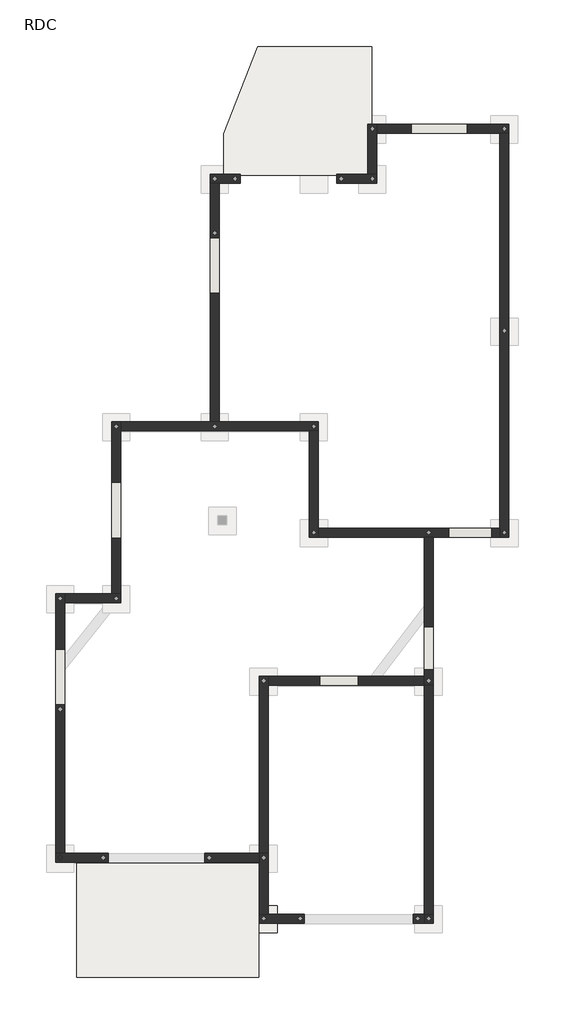
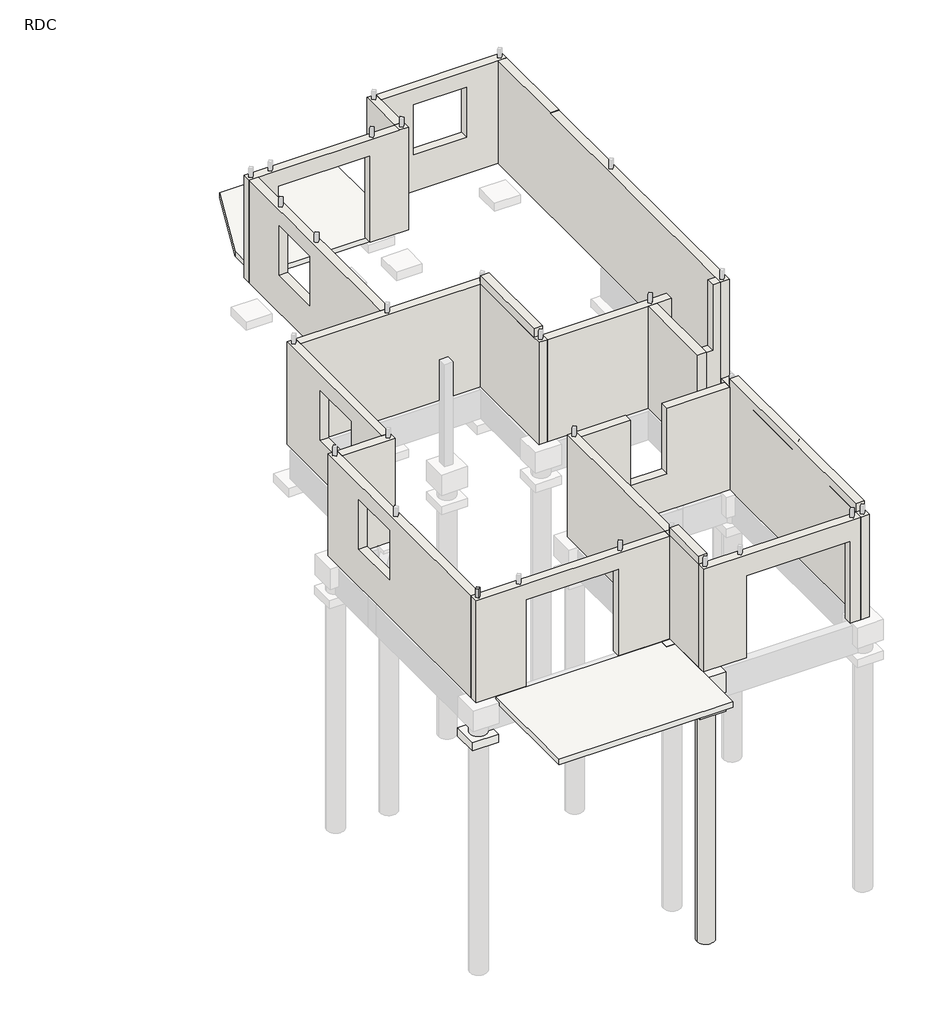
# One storey, part 1 of 5: 20 walls, 5 slabs, 1 column.
"""IFC4 building model written with IfcOpenShell, lengths in millimetres."""

import ifcopenshell
import ifcopenshell.guid

model = None  # the IFC model being written
_history = None  # IfcOwnerHistory: only IFC2X3 demands one
_inside = {}  # id of a spatial element -> (the spatial element, [elements in it])
_under = {}  # id of a project, library or spatial element -> (it, [spatial elements below it])
_declared = {}  # id of a project -> (the project, [libraries it declares])
_typed = {}  # id of a type object -> (the type object, [elements of that type])
_made_of = {}  # id of a material, layer set ... -> (it, [elements and type objects made of it])


def new_model(schema):
    """Start an empty IFC model of exactly this schema.

    Asked for "IFC4X3", IfcOpenShell would pick the latest addendum, in which some entities
    have other attributes; the version numbers below select the first issue.
    IFC2X3 requires an IfcOwnerHistory on every rooted entity: one is made here for all.
    """
    global model, _history
    if schema == "IFC4X3":
        model = ifcopenshell.file(schema_version=(4, 3, 0, 0))
    else:
        model = ifcopenshell.file(schema=schema)
    _inside.clear()
    _under.clear()
    _declared.clear()
    _typed.clear()
    _made_of.clear()
    _history = None
    if model.schema == "IFC2X3":
        org = make("IfcOrganization", Name="unknown")
        user = make(
            "IfcPersonAndOrganization",
            ThePerson=make("IfcPerson", FamilyName="unknown"),
            TheOrganization=org,
        )
        app = make(
            "IfcApplication",
            ApplicationDeveloper=org,
            Version="unknown",
            ApplicationFullName="unknown",
            ApplicationIdentifier="unknown",
        )
        _history = make(
            "IfcOwnerHistory",
            OwningUser=user,
            OwningApplication=app,
            ChangeAction="ADDED",
            CreationDate=0,
        )
    return model


def make(cls, **values):
    """One entity of the class cls with the attributes given. An attribute that is None is left unset."""
    return model.create_entity(
        cls, **{name: value for name, value in values.items() if value is not None}
    )


def rooted(cls, **values):
    """An entity with a GlobalId (a new one), such as an element, a storey or a relation."""
    return make(cls, GlobalId=ifcopenshell.guid.new(), OwnerHistory=_history, **values)


def si_unit(unit_type, name, prefix=None):
    """IfcSIUnit, for example si_unit("LENGTHUNIT", "METRE", prefix="MILLI")."""
    return make("IfcSIUnit", UnitType=unit_type, Prefix=prefix, Name=name)


def assignment(units):
    """IfcUnitAssignment: the units of a project."""
    return None if units is None else make("IfcUnitAssignment", Units=units)


def point(xyz):
    """IfcCartesianPoint."""
    return None if xyz is None else make("IfcCartesianPoint", Coordinates=xyz)


def direction(xyz):
    """IfcDirection."""
    return None if xyz is None else make("IfcDirection", DirectionRatios=xyz)


def frame(location, z_axis=None, x_axis=None):
    """IfcAxis2Placement3D, a coordinate frame: its origin and axes. An axis left out is left unset."""
    return make(
        "IfcAxis2Placement3D",
        Location=point(location),
        Axis=direction(z_axis),
        RefDirection=direction(x_axis),
    )


def origin():
    """The frame at (0, 0, 0) with its axes left unset."""
    return frame((0.0, 0.0, 0.0))


def origin_with_axes():
    """The frame at (0, 0, 0) with the z axis (0, 0, 1) and the x axis (1, 0, 0) written out."""
    return frame((0.0, 0.0, 0.0), z_axis=(0.0, 0.0, 1.0), x_axis=(1.0, 0.0, 0.0))


def place(relative_to, where):
    """IfcLocalPlacement: puts the frame where relative to a parent placement (None: the world)."""
    return make(
        "IfcLocalPlacement", PlacementRelTo=relative_to, RelativePlacement=where
    )


def context(
    kind, dimensions, precision=None, world=None, true_north=None, identifier=None
):
    """IfcGeometricRepresentationContext, for example the 3D "Model" context."""
    return make(
        "IfcGeometricRepresentationContext",
        ContextIdentifier=identifier,
        ContextType=kind,
        CoordinateSpaceDimension=dimensions,
        Precision=precision,
        WorldCoordinateSystem=world,
        TrueNorth=true_north,
    )


def project(units=None, contexts=None):
    """IfcProject with its units and contexts."""
    return rooted(
        "IfcProject",
        Name="project",
        RepresentationContexts=contexts,
        UnitsInContext=assignment(units),
    )


def spatial(cls, under=None, at=None, **own):
    """A site, building, storey or space (cls), placed at a placement, below another one or the project."""
    s = rooted(cls, ObjectPlacement=at, **own)
    if under is not None:
        _under.setdefault(under.id(), (under, []))[1].append(s)
    return s


def polyline(points):
    """IfcPolyline through the points."""
    return make("IfcPolyline", Points=[point(p) for p in points])


def circle_curve(where, radius):
    """IfcCircle in the frame where."""
    return make("IfcCircle", Position=where, Radius=radius)


def outline(outer, holes=None, kind="AREA"):
    """IfcArbitraryClosedProfileDef: a profile drawn as a closed curve; with holes, ...WithVoids."""
    if holes is None:
        return make("IfcArbitraryClosedProfileDef", ProfileType=kind, OuterCurve=outer)
    return make(
        "IfcArbitraryProfileDefWithVoids",
        ProfileType=kind,
        OuterCurve=outer,
        InnerCurves=holes,
    )


def extrude(swept, where, along, depth):
    """IfcExtrudedAreaSolid: the profile swept, set in the frame where, extruded along a direction by depth."""
    return make(
        "IfcExtrudedAreaSolid",
        SweptArea=swept,
        Position=where,
        ExtrudedDirection=direction(along),
        Depth=depth,
    )


def faces_of(points, faces, orient=None, outer=None):
    """IfcFace entities. A face is a list of loops; a loop is a list of indices into points, from 0.

    orient and outer hold one flag for each loop. By default every Orientation is true, the
    first loop of a face is its IfcFaceOuterBound and the others are IfcFaceBound.
    """
    made = []
    for i, loops in enumerate(faces):
        bounds = []
        for j, loop in enumerate(loops):
            is_outer = j == 0 if outer is None else outer[i][j]
            bounds.append(
                make(
                    "IfcFaceOuterBound" if is_outer else "IfcFaceBound",
                    Bound=make("IfcPolyLoop", Polygon=[points[k] for k in loop]),
                    Orientation=True if orient is None else orient[i][j],
                )
            )
        made.append(make("IfcFace", Bounds=bounds))
    return made


def faceted_brep(points, faces, orient=None, outer=None, voids=None):
    """IfcFacetedBrep: a solid bounded by flat faces; with voids (closed shells), ...WithVoids."""
    shared = [point(p) for p in points]
    hull = make("IfcClosedShell", CfsFaces=faces_of(shared, faces, orient, outer))
    if voids is None:
        return make("IfcFacetedBrep", Outer=hull)
    return make(
        "IfcFacetedBrepWithVoids",
        Outer=hull,
        Voids=[
            make(cls, CfsFaces=faces_of(shared, fs, o, b)) for cls, fs, o, b in voids
        ],
    )


def shape(context_of_items, identifier, shape_type, items):
    """IfcShapeRepresentation: the items that make up one representation, for example the "Body"."""
    return make(
        "IfcShapeRepresentation",
        ContextOfItems=context_of_items,
        RepresentationIdentifier=identifier,
        RepresentationType=shape_type,
        Items=items,
    )


def made_of(thing, what):
    """Note that an element or type object is made of a material, layer set ...; save() writes the relation."""
    if what is not None:
        _made_of.setdefault(what.id(), (what, []))[1].append(thing)
    return thing


def element(
    cls,
    number,
    at=None,
    inside=None,
    cuts=None,
    type_object=None,
    material=None,
    context=None,
    identifier="Body",
    shape_type=None,
    held_by="IfcProductDefinitionShape",
    body=None,
    shapes=None,
    **own,
):
    """One element of the class cls, such as IfcWall. Its Tag is "e" and its number.

    at: its placement. inside: the storey or other place that contains it. cuts: it is an
    opening in that element (IfcRelVoidsElement). A single representation is given by context,
    identifier, shape_type and body (its items); several are given by shapes. held_by: the class
    of the entity that holds the representations. save() writes the other relations.
    """
    e = rooted(cls, Tag="e%d" % number, ObjectPlacement=at, **own)
    if body is not None:
        shapes = [shape(context, identifier, shape_type, body)]
    if shapes is not None:
        e.Representation = make(held_by, Representations=shapes)
    if inside is not None:
        _inside.setdefault(inside.id(), (inside, []))[1].append(e)
    if cuts is not None:
        rooted(
            "IfcRelVoidsElement", RelatingBuildingElement=cuts, RelatedOpeningElement=e
        )
    if type_object is not None:
        _typed.setdefault(type_object.id(), (type_object, []))[1].append(e)
    return made_of(e, material)


def aggregate(whole, parts):
    """IfcRelAggregates: a whole, such as a stair, and the parts it consists of."""
    return rooted("IfcRelAggregates", RelatingObject=whole, RelatedObjects=parts)


def save(model, path):
    """Write the relations noted so far, then the file.

    IfcRelAggregates (storeys below a building ...), IfcRelContainedInSpatialStructure (elements
    in a storey), IfcRelDefinesByType, IfcRelAssociatesMaterial and IfcRelDeclares: one each for
    every whole, place, type object, material and project.
    """
    for whole, parts in _under.values():
        aggregate(whole, parts)
    for where, things in _inside.values():
        rooted(
            "IfcRelContainedInSpatialStructure",
            RelatedElements=things,
            RelatingStructure=where,
        )
    for kind, things in _typed.values():
        rooted("IfcRelDefinesByType", RelatedObjects=things, RelatingType=kind)
    for what, things in _made_of.values():
        rooted("IfcRelAssociatesMaterial", RelatedObjects=things, RelatingMaterial=what)
    for by, libraries in _declared.values():
        rooted("IfcRelDeclares", RelatingContext=by, RelatedDefinitions=libraries)
    model.write(path)


def plane_surface(at):
    """IfcPlane: the flat surface through the origin of the frame at, square to its z axis."""
    return make("IfcPlane", Position=at)


def cylinder_surface(at, radius):
    """IfcCylindricalSurface: all points at the distance radius from the z axis of the frame at."""
    return make("IfcCylindricalSurface", Position=at, Radius=radius)


def advanced_brep(points, edges, surfaces, faces):
    """IfcAdvancedBrep: a solid bounded by faces that lie on surfaces and meet in shared edges.

    An edge is (start, end): straight between two places in points (the first is 0);
    or (start, end, curve); or (start, end, curve, False) where it runs against its curve.
    A face is (place in surfaces, loops), or (place, loops, False) where it looks against
    its surface's normal. A loop lists edges by number (the first is 1), with a minus sign
    where the edge is run from its end to its start. The first loop is the outer one.
    """
    corners = [point(p) for p in points]
    vertices = [make("IfcVertexPoint", VertexGeometry=c) for c in corners]
    made = []
    for start, end, *more in edges:
        made.append(
            make(
                "IfcEdgeCurve",
                EdgeStart=vertices[start],
                EdgeEnd=vertices[end],
                EdgeGeometry=more[0] if more else make("IfcPolyline", Points=[corners[start], corners[end]]),
                SameSense=more[1] if len(more) > 1 else True,
            )
        )
    hull = []
    for where, loops, *sense in faces:
        bounds = []
        for j, loop in enumerate(loops):
            ring = [make("IfcOrientedEdge", EdgeElement=made[abs(k) - 1], Orientation=k > 0) for k in loop]
            bounds.append(
                make(
                    "IfcFaceOuterBound" if j == 0 else "IfcFaceBound",
                    Bound=make("IfcEdgeLoop", EdgeList=ring),
                    Orientation=True,
                )
            )
        hull.append(make("IfcAdvancedFace", Bounds=bounds, FaceSurface=surfaces[where], SameSense=sense[0] if sense else True))
    return make("IfcAdvancedBrep", Outer=make("IfcClosedShell", CfsFaces=hull))


model = new_model("IFC4")

# Units and contexts
model_context = context("Model", 3, world=origin())
ifc_project = project(units=[si_unit("LENGTHUNIT", "METRE", prefix="MILLI")], contexts=[model_context])

# Site, building, storey
site = spatial("IfcSite", under=ifc_project)
building = spatial("IfcBuilding", under=site)
storey = spatial("IfcBuildingStorey", under=building, Name="RDC", Elevation=0.0)

# Column
placement = place(None, origin())
element("IfcColumn", 1, ObjectType="CV : CV", at=placement, inside=storey, context=model_context, shape_type="Brep", body=[
    faceted_brep([(-6146.4904447, -6595.6690755, 2710.0), (-6199.5234533, -6648.7020841, 2710.0), (-6146.4904447, -6701.7350927, 2710.0), (-6093.4574361, -6648.7020841, 2710.0), (-6146.4904447, -6595.6690755, 0.0), (-6093.4574361, -6648.7020841, 0.0), (-6146.4904447, -6701.7350927, 0.0), (-6199.5234533, -6648.7020841, 0.0), (-6146.4904447, -6595.6690755, 2500.0), (-6199.5234533, -6648.7020841, 2500.0), (-6146.4904447, -6701.7350927, 2500.0), (-6093.4574361, -6648.7020841, 2500.0)], [[[0, 1, 2, 3]], [[4, 5, 6, 7]], [[1, 0, 8, 4, 7, 9]], [[2, 1, 9, 7, 6, 10]], [[3, 2, 10, 6, 5, 11]], [[0, 3, 11, 5, 4, 8]]]),
    faceted_brep([(-6093.4574361, -6648.7020841, 2710.0), (-6146.4904447, -6595.6690755, 2710.0), (-6199.5234533, -6648.7020841, 2710.0), (-6146.4904447, -6701.7350927, 2710.0), (-6093.4574361, -6648.7020841, 0.0), (-6146.4904447, -6701.7350927, 0.0), (-6199.5234533, -6648.7020841, 0.0), (-6146.4904447, -6595.6690755, 0.0), (-6093.4574361, -6648.7020841, 2500.0), (-6146.4904447, -6595.6690755, 2500.0), (-6199.5234533, -6648.7020841, 2500.0), (-6146.4904447, -6701.7350927, 2500.0)], [[[0, 1, 2, 3]], [[4, 5, 6, 7]], [[1, 0, 8, 4, 7, 9]], [[2, 1, 9, 7, 6, 10]], [[3, 2, 10, 6, 5, 11]], [[0, 3, 11, 5, 4, 8]]]),
])

# Slabs
element("IfcSlab", 2, ObjectType="Pieu-Conduite en acier : Diamètre de 400 mm", at=placement, inside=storey, context=model_context, shape_type="AdvancedBrep", body=[
    advanced_brep(
    [(-1866.4904447, -8001.9775185, -6600.0), (-1466.4904447, -8001.9775185, -6600.0), (-1866.4904447, -8001.9775185, -970.0), (-1466.4904447, -8001.9775185, -970.0)],
    [
        (0, 1, circle_curve(frame((-1666.4904447, -8001.9775185, -6600.0), z_axis=(0.0, 0.0, -1.0), x_axis=(1.0, 0.0, 0.0)), 200.0)),
        (1, 0, circle_curve(frame((-1666.4904447, -8001.9775185, -6600.0), z_axis=(0.0, 0.0, -1.0), x_axis=(1.0, 0.0, 0.0)), 200.0)),
        (2, 3, circle_curve(frame((-1666.4904447, -8001.9775185, -970.0), z_axis=(0.0, 0.0, 1.0), x_axis=(1.0, 0.0, 0.0)), 200.0)),
        (3, 2, circle_curve(frame((-1666.4904447, -8001.9775185, -970.0), z_axis=(0.0, 0.0, 1.0), x_axis=(1.0, 0.0, 0.0)), 200.0)),
        (1, 3),
        (2, 0),
    ],
    [
        plane_surface(frame((-1466.4904447, -8001.9775185, -6600.0), z_axis=(0.0, 0.0, -1.0), x_axis=(0.0, -1.0, 0.0))),
        plane_surface(frame((-1969.9771566, -7701.9775185, -970.0), z_axis=(0.0, 0.0, 1.0), x_axis=(1.0, 0.0, 0.0))),
        cylinder_surface(frame((-1666.4904447, -8001.9775185, -6600.0), z_axis=(0.0, 0.0, 1.0), x_axis=(1.0, 0.0, 0.0)), 200.0),
    ],
    [
        (0, [[1, 2]]),
        (1, [[3, 4]]),
        (2, [[-2, 5, -3, 6]]),
        (2, [[-1, -6, -4, -5]]),
    ],
),
    advanced_brep(
    [(-1866.4904447, -8001.9775185, -770.0), (-1466.4904447, -8001.9775185, -770.0), (-1466.4904447, -8001.9775185, -500.0), (-1493.285364, -8101.9775185, -500.0), (-1866.4904447, -8001.9775185, -500.0), (-1766.4904447, -7828.7724377, -500.0), (-1566.4904447, -7828.7724377, -500.0), (-1493.2937812, -7901.9629409, -500.0)],
    [
        (0, 1, circle_curve(frame((-1666.4904447, -8001.9775185, -770.0), z_axis=(0.0, 0.0, 1.0), x_axis=(1.0, 0.0, 0.0)), 200.0)),
        (1, 2),
        (2, 3, circle_curve(frame((-1666.4904447, -8001.9775185, -500.0), z_axis=(0.0, 0.0, -1.0), x_axis=(1.0, 0.0, 0.0)), 200.0)),
        (3, 4, circle_curve(frame((-1666.4904447, -8001.9775185, -500.0), z_axis=(0.0, 0.0, -1.0), x_axis=(1.0, 0.0, 0.0)), 200.0)),
        (4, 0),
        (1, 0, circle_curve(frame((-1666.4904447, -8001.9775185, -770.0), z_axis=(0.0, 0.0, 1.0), x_axis=(1.0, 0.0, 0.0)), 200.0)),
        (4, 5, circle_curve(frame((-1666.4904447, -8001.9775185, -500.0), z_axis=(0.0, 0.0, -1.0), x_axis=(1.0, 0.0, 0.0)), 200.0)),
        (5, 6, circle_curve(frame((-1666.4904447, -8001.9775185, -500.0), z_axis=(0.0, 0.0, -1.0), x_axis=(1.0, 0.0, 0.0)), 200.0)),
        (6, 7, circle_curve(frame((-1666.4904447, -8001.9775185, -500.0), z_axis=(0.0, 0.0, -1.0), x_axis=(1.0, 0.0, 0.0)), 200.0)),
        (7, 2, circle_curve(frame((-1666.4904447, -8001.9775185, -500.0), z_axis=(0.0, 0.0, -1.0), x_axis=(1.0, 0.0, 0.0)), 200.0)),
    ],
    [
        cylinder_surface(frame((-1666.4904447, -8001.9775185, -6600.0), z_axis=(0.0, 0.0, 1.0), x_axis=(1.0, 0.0, 0.0)), 200.0),
        plane_surface(frame((-1969.9771566, -7701.9775185, -770.0), z_axis=(0.0, 0.0, -1.0), x_axis=(-1.0, 0.0, 0.0))),
        plane_surface(frame((-1966.4904447, -7701.9775185, -500.0), z_axis=(0.0, 0.0, 1.0), x_axis=(1.0, 0.0, 0.0))),
    ],
    [
        (0, [[1, 2, 3, 4, 5]]),
        (0, [[6, -5, 7, 8, 9, 10, -2]]),
        (1, [[-1, -6]]),
        (2, [[-4, -3, -10, -9, -8, -7]]),
    ],
),
])
element("IfcSlab", 3, ObjectType="Dalla BA 13", at=placement, inside=storey, context=model_context, shape_type="SweptSolid", body=[
    extrude(outline(polyline([(-2545.6685695, 9313.5020686), (-1792.0228909, 11240.4191575), (720.0228632, 11240.4191575), (720.0228632, 9513.5020686), (630.0228631, 9513.5020686), (630.0228631, 8408.0224784), (-2545.6685695, 8408.0224784), (-2545.6685695, 9313.5020686)])), frame((0.0, 0.0, -130.0), z_axis=(0.0, 0.0, 1.0), x_axis=(1.0, 0.0, 0.0)), (0.0, 0.0, 1.0), 130.0),
    extrude(outline(polyline([(-1769.9771448, -6761.9775197), (-1769.9771448, -9284.514976), (-5789.9771448, -9284.514976), (-5789.9771448, -6761.9775197), (-1769.9771448, -6761.9775197)])), frame((0.0, 0.0, -130.0), z_axis=(0.0, 0.0, 1.0), x_axis=(1.0, 0.0, 0.0)), (0.0, 0.0, 1.0), 130.0),
])
element("IfcSlab", 4, ObjectType="Tête de pieux-1 poteau : 60x60x50", at=placement, inside=storey, context=model_context, shape_type="Brep", body=[
    faceted_brep([(-1366.4904447, -7701.9775185, 0.0), (-1966.4904447, -7701.9775185, 0.0), (-1966.4904447, -8301.9775185, 0.0), (-1366.4904447, -8301.9775185, 0.0), (-1366.4904447, -7701.9775185, -500.0), (-1366.4904447, -7901.9775185, -500.0), (-1366.4904447, -8101.9775185, -500.0), (-1366.4904447, -8301.9775185, -500.0), (-1966.4904447, -8301.9775185, -500.0), (-1966.4904447, -7701.9775185, -500.0), (-1766.4904447, -7701.9775185, -500.0), (-1566.4904447, -7701.9775185, -500.0)], [[[0, 1, 2, 3]], [[4, 5, 6, 7, 8, 9, 10, 11]], [[1, 0, 4, 11, 10, 9]], [[2, 1, 9, 8]], [[3, 2, 8, 7]], [[0, 3, 7, 6, 5, 4]]]),
])
element("IfcSlab", 5, ObjectType="M_Base-Rectangulaire : 60x60x20", at=placement, inside=storey, context=model_context, shape_type="SweptSolid", body=[
    extrude(outline(polyline([(-1369.9771566, -7701.9775185), (-1369.9771566, -8301.9775185), (-1969.9771566, -8301.9775185), (-1969.9771566, -7701.9775185), (-1369.9771566, -7701.9775185)])), frame((0.0, 0.0, -970.0), z_axis=(0.0, 0.0, 1.0), x_axis=(1.0, 0.0, 0.0)), (0.0, 0.0, 1.0), 200.0),
    extrude(outline(polyline([(-1369.9771566, -7701.9775185), (-1369.9771566, -8301.9775185), (-1969.9771566, -8301.9775185), (-1969.9771566, -7701.9775185), (-1369.9771566, -7701.9775185)])), frame((0.0, 0.0, -970.0), z_axis=(0.0, 0.0, 1.0), x_axis=(1.0, 0.0, 0.0)), (0.0, 0.0, 1.0), 200.0),
])
element("IfcSlab", 6, ObjectType="M_Base-Rectangulaire : 60x60x20", at=placement, inside=storey, context=model_context, shape_type="SweptSolid", body=[
    extrude(outline(polyline([(-5851.0339778, -6364.5149728), (-5851.0339778, -6964.5149728), (-6451.0339778, -6964.5149728), (-6451.0339778, -6364.5149728), (-5851.0339778, -6364.5149728)])), frame((0.0, 0.0, -970.0), z_axis=(0.0, 0.0, 1.0), x_axis=(1.0, 0.0, 0.0)), (0.0, 0.0, 1.0), 200.0),
    extrude(outline(polyline([(-5851.0339778, -6364.5149728), (-5851.0339778, -6964.5149728), (-6451.0339778, -6964.5149728), (-6451.0339778, -6364.5149728), (-5851.0339778, -6364.5149728)])), frame((0.0, 0.0, -970.0), z_axis=(0.0, 0.0, 1.0), x_axis=(1.0, 0.0, 0.0)), (0.0, 0.0, 1.0), 200.0),
])

# Walls
element("IfcWall", 7, ObjectType="Briques 20cm", at=placement, inside=storey, context=model_context, shape_type="Brep", body=[
    faceted_brep([(-50.4336241, 8223.8353965, 2115.0), (-50.4336241, 8223.8353965, 0.0), (834.5663962, 8223.8353965, 0.0), (834.5663962, 8223.8353965, 2510.0), (634.5663962, 8223.8353965, 2510.0), (634.5663962, 8223.8353965, 2500.0), (-2645.4336004, 8223.8353965, 2500.0), (-2845.4336004, 8223.8353965, 2500.0), (-2845.4336004, 8223.8353965, 0.0), (-2645.4336004, 8223.8353965, 0.0), (-2180.4336241, 8223.8353965, 0.0), (-2180.4336241, 8223.8353965, 2115.0), (-50.4336241, 8423.8353965, 0.0), (-50.4336241, 8423.8353965, 2115.0), (-2180.4336241, 8423.8353965, 2115.0), (-2180.4336241, 8423.8353965, 0.0), (-2845.4336004, 8423.8353965, 0.0), (-2845.4336004, 8423.8353965, 2500.0), (634.5663962, 8423.8353965, 2500.0), (634.5663962, 8423.8353965, 2510.0), (834.5663962, 8423.8353965, 2510.0), (834.5663962, 8423.8353965, 0.0), (634.5663962, 8423.8353965, 0.0), (787.5993877, 8323.8353965, 0.0), (734.5663791, 8376.8684051, 0.0), (681.5333706, 8323.8353965, 0.0), (734.5663791, 8270.8023879, 0.0), (102.5994047, 8323.8353965, 0.0), (49.5663962, 8376.8684051, 0.0), (-3.4666124, 8323.8353965, 0.0), (49.5663962, 8270.8023879, 0.0), (-2242.4005953, 8323.8353965, 0.0), (-2295.4336038, 8376.8684051, 0.0), (-2348.4666124, 8323.8353965, 0.0), (-2295.4336038, 8270.8023879, 0.0), (-2692.4005918, 8323.8353965, 0.0), (-2745.4336004, 8376.8684051, 0.0), (-2798.466609, 8323.8353965, 0.0), (-2745.4336004, 8270.8023879, 0.0), (787.5993877, 8323.8353965, 2510.0), (734.5663791, 8376.8684051, 2510.0), (681.5333706, 8323.8353965, 2510.0), (734.5663791, 8270.8023879, 2510.0), (102.5994047, 8323.8353965, 2500.0), (49.5663962, 8376.8684051, 2500.0), (-3.4666124, 8323.8353965, 2500.0), (49.5663962, 8270.8023879, 2500.0), (-2242.4005953, 8323.8353965, 2500.0), (-2295.4336038, 8376.8684051, 2500.0), (-2348.4666124, 8323.8353965, 2500.0), (-2295.4336038, 8270.8023879, 2500.0), (-2692.4005918, 8323.8353965, 2500.0), (-2745.4336004, 8376.8684051, 2500.0), (-2798.466609, 8323.8353965, 2500.0), (-2745.4336004, 8270.8023879, 2500.0)], [[[0, 1, 2, 3, 4, 5, 6, 7, 8, 9, 10, 11]], [[12, 13, 14, 15, 16, 17, 18, 19, 20, 21, 22]], [[21, 2, 1, 12, 22], [23, 24, 25, 26], [27, 28, 29, 30]], [[15, 10, 9, 8, 16], [31, 32, 33, 34], [35, 36, 37, 38]], [[2, 21, 20, 3]], [[1, 0, 13, 12]], [[11, 10, 15, 14]], [[0, 11, 14, 13]], [[24, 23, 39, 40]], [[25, 24, 40, 41]], [[26, 25, 41, 42]], [[23, 26, 42, 39]], [[28, 27, 43, 44]], [[29, 28, 44, 45]], [[30, 29, 45, 46]], [[27, 30, 46, 43]], [[32, 31, 47, 48]], [[33, 32, 48, 49]], [[34, 33, 49, 50]], [[31, 34, 50, 47]], [[36, 35, 51, 52]], [[37, 36, 52, 53]], [[38, 37, 53, 54]], [[35, 38, 54, 51]], [[16, 8, 7, 17]], [[5, 18, 17, 7, 6], [44, 43, 46, 45], [48, 47, 50, 49], [52, 51, 54, 53]], [[18, 5, 4, 19]], [[4, 3, 20, 19], [40, 39, 42, 41]]]),
])
element("IfcWall", 8, ObjectType="Briques 20cm", at=placement, inside=storey, context=model_context, shape_type="Brep", body=[
    faceted_brep([(834.5663962, 8423.8353965, 0.0), (834.5663962, 9329.3149644, 0.0), (834.5663962, 9529.3149644, 0.0), (834.5663962, 9529.3149644, 2510.0), (834.5663962, 9329.3149644, 2510.0), (834.5663962, 8423.8353965, 2510.0), (634.5663962, 9529.3149644, 0.0), (634.5663962, 8423.8353965, 0.0), (634.5663962, 8423.8353965, 2500.0), (634.5663962, 8423.8353965, 2510.0), (634.5663962, 9529.3149644, 2510.0), (787.5993877, 9429.3149644, 0.0), (734.5663791, 9482.347973, 0.0), (681.5333706, 9429.3149644, 0.0), (734.5663791, 9376.2819558, 0.0), (787.5993877, 9429.3149644, 2510.0), (734.5663791, 9482.347973, 2510.0), (681.5333706, 9429.3149644, 2510.0), (734.5663791, 9376.2819558, 2510.0)], [[[0, 1, 2, 3, 4, 5]], [[6, 7, 8, 9, 10]], [[2, 1, 0, 7, 6], [11, 12, 13, 14]], [[7, 0, 5, 9, 8]], [[2, 6, 10, 3]], [[12, 11, 15, 16]], [[13, 12, 16, 17]], [[14, 13, 17, 18]], [[11, 14, 18, 15]], [[5, 4, 3, 10, 9], [16, 15, 18, 17]]]),
])
element("IfcWall", 9, ObjectType="Briques 20cm", at=placement, inside=storey, context=model_context, shape_type="Brep", body=[
    faceted_brep([(834.5663962, 9329.3149644, 0.0), (3544.5663998, 9329.3149644, 0.0), (3744.5663998, 9329.3149644, 0.0), (3744.5663998, 9329.3149644, 2510.0), (3544.5663998, 9329.3149644, 2510.0), (834.5663962, 9329.3149644, 2510.0), (2819.5663803, 9329.3149644, 2115.0), (2819.5663803, 9329.3149644, 900.0), (1589.5663803, 9329.3149644, 900.0), (1589.5663803, 9329.3149644, 2115.0), (3744.5663998, 9529.3149644, 0.0), (834.5663962, 9529.3149644, 0.0), (834.5663962, 9529.3149644, 2510.0), (3744.5663998, 9529.3149644, 2510.0), (2819.5663803, 9529.3149644, 900.0), (2819.5663803, 9529.3149644, 2115.0), (1589.5663803, 9529.3149644, 2115.0), (1589.5663803, 9529.3149644, 900.0), (3697.5994084, 9429.3149644, 0.0), (3644.5663998, 9482.347973, 0.0), (3591.5333912, 9429.3149644, 0.0), (3644.5663998, 9376.2819558, 0.0), (3697.5994084, 9429.3149644, 2510.0), (3644.5663998, 9482.347973, 2510.0), (3591.5333912, 9429.3149644, 2510.0), (3644.5663998, 9376.2819558, 2510.0)], [[[0, 1, 2, 3, 4, 5], [6, 7, 8, 9]], [[10, 11, 12, 13], [14, 15, 16, 17]], [[2, 1, 0, 11, 10], [18, 19, 20, 21]], [[11, 0, 5, 12]], [[2, 10, 13, 3]], [[7, 6, 15, 14]], [[8, 7, 14, 17]], [[9, 8, 17, 16]], [[6, 9, 16, 15]], [[19, 18, 22, 23]], [[20, 19, 23, 24]], [[21, 20, 24, 25]], [[18, 21, 25, 22]], [[5, 4, 3, 13, 12], [23, 22, 25, 24]]]),
])
element("IfcWall", 10, ObjectType="Briques 20cm", at=placement, inside=storey, context=model_context, shape_type="Brep", body=[
    faceted_brep([(3544.5663998, 9329.3149644, 0.0), (3544.5663998, 623.8353756, 0.0), (3544.5663998, 423.8353756, 0.0), (3544.5663998, 423.8353756, 2500.0), (3544.5663998, 623.8353756, 2500.0), (3544.5663998, 7232.9791151, 2500.0), (3544.5663998, 7232.9791151, 2510.0), (3544.5663998, 9329.3149644, 2510.0), (3744.5663998, 423.8353756, 0.0), (3744.5663998, 9329.3149644, 0.0), (3744.5663998, 9329.3149644, 2510.0), (3744.5663998, 7232.9791151, 2510.0), (3744.5663998, 7232.9791151, 2500.0), (3744.5663998, 423.8353756, 2500.0), (3697.5994084, 523.8353673, 0.0), (3644.5663998, 576.8683759, 0.0), (3591.5333912, 523.8353673, 0.0), (3644.5663998, 470.8023588, 0.0), (3697.5994084, 4974.3149644, 0.0), (3644.5663998, 5027.347973, 0.0), (3591.5333912, 4974.3149644, 0.0), (3644.5663998, 4921.2819558, 0.0), (3697.5994084, 523.8353673, 2500.0), (3644.5663998, 576.8683759, 2500.0), (3591.5333912, 523.8353673, 2500.0), (3644.5663998, 470.8023588, 2500.0), (3697.5994084, 4974.3149644, 2500.0), (3644.5663998, 5027.347973, 2500.0), (3591.5333912, 4974.3149644, 2500.0), (3644.5663998, 4921.2819558, 2500.0)], [[[0, 1, 2, 3, 4, 5, 6, 7]], [[8, 9, 10, 11, 12, 13]], [[2, 1, 0, 9, 8], [14, 15, 16, 17], [18, 19, 20, 21]], [[9, 0, 7, 10]], [[2, 8, 13, 3]], [[15, 14, 22, 23]], [[16, 15, 23, 24]], [[17, 16, 24, 25]], [[14, 17, 25, 22]], [[19, 18, 26, 27]], [[20, 19, 27, 28]], [[21, 20, 28, 29]], [[18, 21, 29, 26]], [[12, 5, 4, 3, 13], [23, 22, 25, 24], [27, 26, 29, 28]], [[5, 12, 11, 6]], [[7, 6, 11, 10]]]),
])
element("IfcWall", 11, ObjectType="Briques 20cm", at=placement, inside=storey, context=model_context, shape_type="Brep", body=[
    faceted_brep([(3544.5663998, 623.8353756, 0.0), (-455.4335795, 623.8353756, 0.0), (-455.4335795, 623.8353756, 2500.0), (2074.5663809, 623.8353756, 2500.0), (2414.643182, 623.8353756, 2500.0), (2414.643182, 623.8353756, 900.0), (3364.643182, 623.8353756, 900.0), (3364.643182, 623.8353756, 2500.0), (3544.5663998, 623.8353756, 2500.0), (-455.4335795, 423.8353756, 0.0), (1874.5663809, 423.8353756, 0.0), (2074.5663809, 423.8353756, 0.0), (3544.5663998, 423.8353756, 0.0), (3544.5663998, 423.8353756, 2500.0), (3364.643182, 423.8353756, 2500.0), (3364.643182, 423.8353756, 900.0), (2414.643182, 423.8353756, 900.0), (2414.643182, 423.8353756, 2500.0), (2074.5663809, 423.8353756, 2500.0), (1874.5663809, 423.8353756, 2500.0), (-455.4335795, 423.8353756, 2500.0), (2027.5993725, 523.8353673, 0.0), (1974.5663639, 576.8683759, 0.0), (1921.5333553, 523.8353673, 0.0), (1974.5663639, 470.8023588, 0.0), (2027.5993725, 523.8353673, 2500.0), (1974.5663639, 576.8683759, 2500.0), (1921.5333553, 523.8353673, 2500.0), (1974.5663639, 470.8023588, 2500.0)], [[[0, 1, 2, 3, 4, 5, 6, 7, 8]], [[9, 10, 11, 12, 13, 14, 15, 16, 17, 18, 19, 20]], [[1, 0, 12, 11, 10, 9], [21, 22, 23, 24]], [[12, 0, 8, 13]], [[1, 9, 20, 2]], [[5, 16, 15, 6]], [[16, 5, 4, 17]], [[6, 15, 14, 7]], [[22, 21, 25, 26]], [[23, 22, 26, 27]], [[24, 23, 27, 28]], [[21, 24, 28, 25]], [[2, 20, 19, 18, 17, 4, 3], [26, 25, 28, 27]], [[8, 7, 14, 13]]]),
])
element("IfcWall", 12, ObjectType="Briques 20cm", at=placement, inside=storey, context=model_context, shape_type="Brep", body=[
    faceted_brep([(-2960.9620445, -6548.702077, 0.0), (-2960.9620445, -6548.702077, 2115.0), (-5090.9620445, -6548.702077, 2115.0), (-5090.9620445, -6548.702077, 0.0), (-6046.490445, -6548.702077, 0.0), (-6246.490445, -6548.702077, 0.0), (-6246.490445, -6548.702077, 2500.0), (-6046.490445, -6548.702077, 2500.0), (-1766.4904447, -6548.702077, 2500.0), (-1766.4904447, -6548.702077, 0.0), (-2960.9620445, -6748.702077, 2115.0), (-2960.9620445, -6748.702077, 0.0), (-1766.4904447, -6748.702077, 0.0), (-1766.4904447, -6748.702077, 2500.0), (-6246.490445, -6748.702077, 2500.0), (-6246.490445, -6748.702077, 0.0), (-5090.9620445, -6748.702077, 0.0), (-5090.9620445, -6748.702077, 2115.0), (-6093.4574361, -6648.7020841, 0.0), (-6146.4904447, -6595.6690755, 0.0), (-6199.5234533, -6648.7020841, 0.0), (-6146.4904447, -6701.7350927, 0.0), (-5144.5884006, -6648.7020841, 0.0), (-5197.6214092, -6595.6690755, 0.0), (-5250.6544178, -6648.7020841, 0.0), (-5197.6214092, -6701.7350927, 0.0), (-2808.4574361, -6648.7020841, 0.0), (-2861.4904447, -6595.6690755, 0.0), (-2914.5234533, -6648.7020841, 0.0), (-2861.4904447, -6701.7350927, 0.0), (-6093.4574361, -6648.7020841, 2500.0), (-6146.4904447, -6595.6690755, 2500.0), (-6199.5234533, -6648.7020841, 2500.0), (-6146.4904447, -6701.7350927, 2500.0), (-5144.5884006, -6648.7020841, 2500.0), (-5197.6214092, -6595.6690755, 2500.0), (-5250.6544178, -6648.7020841, 2500.0), (-5197.6214092, -6701.7350927, 2500.0), (-2808.4574361, -6648.7020841, 2500.0), (-2861.4904447, -6595.6690755, 2500.0), (-2914.5234533, -6648.7020841, 2500.0), (-2861.4904447, -6701.7350927, 2500.0)], [[[0, 1, 2, 3, 4, 5, 6, 7, 8, 9]], [[10, 11, 12, 13, 14, 15, 16, 17]], [[15, 5, 4, 3, 16], [18, 19, 20, 21], [22, 23, 24, 25]], [[9, 12, 11, 0], [26, 27, 28, 29]], [[5, 15, 14, 6]], [[12, 9, 8, 13]], [[11, 10, 1, 0]], [[17, 16, 3, 2]], [[10, 17, 2, 1]], [[19, 18, 30, 31]], [[20, 19, 31, 32]], [[21, 20, 32, 33]], [[18, 21, 33, 30]], [[23, 22, 34, 35]], [[24, 23, 35, 36]], [[25, 24, 36, 37]], [[22, 25, 37, 34]], [[27, 26, 38, 39]], [[28, 27, 39, 40]], [[29, 28, 40, 41]], [[26, 29, 41, 38]], [[8, 7, 6, 14, 13], [31, 30, 33, 32], [35, 34, 37, 36], [39, 38, 41, 40]]]),
])
element("IfcWall", 13, ObjectType="Briques 20cm", at=placement, inside=storey, context=model_context, shape_type="Brep", body=[
    faceted_brep([(-6046.490445, -6548.702077, 0.0), (-6046.490445, -1028.5605284, 0.0), (-6046.490445, -828.5605284, 0.0), (-6046.490445, -828.5605284, 2500.0), (-6046.490445, -1028.5605284, 2500.0), (-6046.490445, -6548.702077, 2500.0), (-6046.490445, -3276.1682683, 900.0), (-6046.490445, -3276.1682683, 2115.0), (-6046.490445, -2046.1682683, 2115.0), (-6046.490445, -2046.1682683, 900.0), (-6246.490445, -828.5605284, 0.0), (-6246.490445, -6548.702077, 0.0), (-6246.490445, -6548.702077, 2500.0), (-6246.490445, -828.5605284, 2500.0), (-6246.490445, -3276.1682683, 2115.0), (-6246.490445, -3276.1682683, 900.0), (-6246.490445, -2046.1682683, 900.0), (-6246.490445, -2046.1682683, 2115.0), (-6093.4574361, -928.5605356, 0.0), (-6146.4904447, -875.527527, 0.0), (-6199.5234533, -928.5605356, 0.0), (-6146.4904447, -981.5935442, 0.0), (-6093.4574361, -3373.5605284, 0.0), (-6146.4904447, -3320.5275198, 0.0), (-6199.5234533, -3373.5605284, 0.0), (-6146.4904447, -3426.593537, 0.0), (-6093.4574361, -928.5605356, 2500.0), (-6146.4904447, -875.527527, 2500.0), (-6199.5234533, -928.5605356, 2500.0), (-6146.4904447, -981.5935442, 2500.0), (-6093.4574361, -3373.5605284, 2500.0), (-6146.4904447, -3320.5275198, 2500.0), (-6199.5234533, -3373.5605284, 2500.0), (-6146.4904447, -3426.593537, 2500.0)], [[[0, 1, 2, 3, 4, 5], [6, 7, 8, 9]], [[10, 11, 12, 13], [14, 15, 16, 17]], [[2, 1, 0, 11, 10], [18, 19, 20, 21], [22, 23, 24, 25]], [[11, 0, 5, 12]], [[2, 10, 13, 3]], [[15, 14, 7, 6]], [[16, 15, 6, 9]], [[17, 16, 9, 8]], [[14, 17, 8, 7]], [[19, 18, 26, 27]], [[20, 19, 27, 28]], [[21, 20, 28, 29]], [[18, 21, 29, 26]], [[23, 22, 30, 31]], [[24, 23, 31, 32]], [[25, 24, 32, 33]], [[22, 25, 33, 30]], [[5, 4, 3, 13, 12], [27, 26, 29, 28], [31, 30, 33, 32]]]),
])
element("IfcWall", 14, ObjectType="Briques 20cm", at=placement, inside=storey, context=model_context, shape_type="Brep", body=[
    faceted_brep([(-6046.490445, -1028.5605284, 0.0), (-4812.6214092, -1028.5605284, 0.0), (-4812.6214092, -1028.5605284, 2500.0), (-6046.490445, -1028.5605284, 2500.0), (-4812.6214092, -828.5605284, 0.0), (-5012.6214092, -828.5605284, 0.0), (-6046.490445, -828.5605284, 0.0), (-6046.490445, -828.5605284, 2500.0), (-5012.6214092, -828.5605284, 2500.0), (-4812.6214092, -828.5605284, 2500.0), (-4859.5884006, -928.5605185, 0.0), (-4912.6214092, -875.52751, 0.0), (-4965.6544178, -928.5605185, 0.0), (-4912.6214092, -981.5935271, 0.0), (-4859.5884006, -928.5605185, 2500.0), (-4912.6214092, -875.52751, 2500.0), (-4965.6544178, -928.5605185, 2500.0), (-4912.6214092, -981.5935271, 2500.0)], [[[0, 1, 2, 3]], [[4, 5, 6, 7, 8, 9]], [[1, 0, 6, 5, 4], [10, 11, 12, 13]], [[6, 0, 3, 7]], [[1, 4, 9, 2]], [[11, 10, 14, 15]], [[12, 11, 15, 16]], [[13, 12, 16, 17]], [[10, 13, 17, 14]], [[3, 2, 9, 8, 7], [15, 14, 17, 16]]]),
])
element("IfcWall", 15, ObjectType="Briques 20cm", at=placement, inside=storey, context=model_context, shape_type="Brep", body=[
    faceted_brep([(-4812.6214092, -828.5605284, 0.0), (-4812.6214092, 2763.8353669, 0.0), (-4812.6214092, 2963.8353669, 0.0), (-4812.6214092, 2963.8353669, 2500.0), (-4812.6214092, 2763.8353669, 2500.0), (-4812.6214092, -828.5605284, 2500.0), (-4812.6214092, 1631.4394925, 2115.0), (-4812.6214092, 1631.4394925, 900.0), (-4812.6214092, 401.4394925, 900.0), (-4812.6214092, 401.4394925, 2115.0), (-5012.6214092, 2963.8353669, 0.0), (-5012.6214092, -828.5605284, 0.0), (-5012.6214092, -828.5605284, 2500.0), (-5012.6214092, 2963.8353669, 2500.0), (-5012.6214092, 1631.4394925, 900.0), (-5012.6214092, 1631.4394925, 2115.0), (-5012.6214092, 401.4394925, 2115.0), (-5012.6214092, 401.4394925, 900.0), (-4859.5884006, 2863.8353669, 0.0), (-4912.6214092, 2916.8683755, 0.0), (-4965.6544178, 2863.8353669, 0.0), (-4912.6214092, 2810.8023583, 0.0), (-4859.5884006, 2863.8353669, 2500.0), (-4912.6214092, 2916.8683755, 2500.0), (-4965.6544178, 2863.8353669, 2500.0), (-4912.6214092, 2810.8023583, 2500.0)], [[[0, 1, 2, 3, 4, 5], [6, 7, 8, 9]], [[10, 11, 12, 13], [14, 15, 16, 17]], [[2, 1, 0, 11, 10], [18, 19, 20, 21]], [[11, 0, 5, 12]], [[2, 10, 13, 3]], [[7, 6, 15, 14]], [[8, 7, 14, 17]], [[9, 8, 17, 16]], [[6, 9, 16, 15]], [[19, 18, 22, 23]], [[20, 19, 23, 24]], [[21, 20, 24, 25]], [[18, 21, 25, 22]], [[5, 4, 3, 13, 12], [23, 22, 25, 24]]]),
])
element("IfcWall", 16, ObjectType="Briques 20cm", at=placement, inside=storey, context=model_context, shape_type="Brep", body=[
    faceted_brep([(-4812.6214092, 2763.8353669, 0.0), (-655.4335795, 2763.8353669, 0.0), (-455.4335795, 2763.8353669, 0.0), (-455.4335795, 2763.8353669, 2500.0), (-655.4335795, 2763.8353669, 2500.0), (-2472.9274976, 2763.8353669, 2500.0), (-4812.6214092, 2763.8353669, 2500.0), (-455.4335795, 2963.8353669, 0.0), (-2645.4336004, 2963.8353669, 0.0), (-2845.4336004, 2963.8353669, 0.0), (-4812.6214092, 2963.8353669, 0.0), (-4812.6214092, 2963.8353669, 2500.0), (-2845.4336004, 2963.8353669, 2500.0), (-2645.4336004, 2963.8353669, 2500.0), (-2472.9274976, 2963.8353669, 2500.0), (-455.4335795, 2963.8353669, 2500.0), (-2692.4005918, 2863.8353669, 0.0), (-2745.4336004, 2916.8683755, 0.0), (-2798.466609, 2863.8353669, 0.0), (-2745.4336004, 2810.8023583, 0.0), (-502.4005879, 2863.8353669, 0.0), (-555.4335965, 2916.8683755, 0.0), (-608.4666051, 2863.8353669, 0.0), (-555.4335965, 2810.8023583, 0.0), (-2692.4005918, 2863.8353669, 2500.0), (-2745.4336004, 2916.8683755, 2500.0), (-2798.466609, 2863.8353669, 2500.0), (-2745.4336004, 2810.8023583, 2500.0), (-502.4005879, 2863.8353669, 2500.0), (-555.4335965, 2916.8683755, 2500.0), (-608.4666051, 2863.8353669, 2500.0), (-555.4335965, 2810.8023583, 2500.0)], [[[0, 1, 2, 3, 4, 5, 6]], [[7, 8, 9, 10, 11, 12, 13, 14, 15]], [[2, 1, 0, 10, 9, 8, 7], [16, 17, 18, 19], [20, 21, 22, 23]], [[10, 0, 6, 11]], [[2, 7, 15, 3]], [[17, 16, 24, 25]], [[18, 17, 25, 26]], [[19, 18, 26, 27]], [[16, 19, 27, 24]], [[21, 20, 28, 29]], [[22, 21, 29, 30]], [[23, 22, 30, 31]], [[20, 23, 31, 28]], [[3, 15, 14, 13, 12, 11, 6, 5, 4], [25, 24, 27, 26], [29, 28, 31, 30]]]),
])
element("IfcWall", 17, ObjectType="Briques 20cm", at=placement, inside=storey, context=model_context, shape_type="Brep", body=[
    faceted_brep([(-655.4335795, 2763.8353669, 0.0), (-655.4335795, 423.8353756, 0.0), (-655.4335795, 423.8353756, 2500.0), (-655.4335795, 697.5075352, 2500.0), (-655.4335795, 2763.8353669, 2500.0), (-455.4335795, 423.8353756, 0.0), (-455.4335795, 623.8353756, 0.0), (-455.4335795, 2763.8353669, 0.0), (-455.4335795, 2763.8353669, 2500.0), (-455.4335795, 697.5075352, 2500.0), (-455.4335795, 623.8353756, 2500.0), (-455.4335795, 423.8353756, 2500.0), (-502.4005879, 523.8353673, 0.0), (-555.4335965, 576.8683759, 0.0), (-608.4666051, 523.8353673, 0.0), (-555.4335965, 470.8023588, 0.0), (-502.4005879, 523.8353673, 2500.0), (-555.4335965, 576.8683759, 2500.0), (-608.4666051, 523.8353673, 2500.0), (-555.4335965, 470.8023588, 2500.0)], [[[0, 1, 2, 3, 4]], [[5, 6, 7, 8, 9, 10, 11]], [[1, 0, 7, 6, 5], [12, 13, 14, 15]], [[7, 0, 4, 8]], [[1, 5, 11, 2]], [[13, 12, 16, 17]], [[14, 13, 17, 18]], [[15, 14, 18, 19]], [[12, 15, 19, 16]], [[2, 11, 10, 9, 8, 4, 3], [17, 16, 19, 18]]]),
])
element("IfcWall", 18, ObjectType="Briques 20cm", at=placement, inside=storey, context=model_context, shape_type="SweptSolid", body=[
    extrude(outline(polyline([(0.0, -1566.4904447), (0.0, 1874.5663809), (2500.0, 1874.5663809), (2500.0, 422.303338), (900.0, 422.303338), (900.0, -427.696662), (2500.0, -427.696662), (2500.0, -1566.4904447), (0.0, -1566.4904447)])), frame((0.0, -2846.1646234, 0.0), z_axis=(0.0, 1.0, 0.0), x_axis=(0.0, 0.0, 1.0)), (0.0, 0.0, 1.0), 200.0),
])
element("IfcWall", 19, ObjectType="Briques 20cm", at=placement, inside=storey, context=model_context, shape_type="Brep", body=[
    faceted_brep([(-1566.4904447, -6548.702077, 0.0), (-1566.4904447, -2846.1646234, 0.0), (-1566.4904447, -2646.1646234, 0.0), (-1566.4904447, -2646.1646234, 2500.0), (-1566.4904447, -2846.1646234, 2500.0), (-1566.4904447, -6548.702077, 2500.0), (-1766.4904447, -2646.1646234, 0.0), (-1766.4904447, -6548.702077, 0.0), (-1766.4904447, -6548.702077, 2500.0), (-1766.4904447, -2646.1646234, 2500.0), (-1612.400632, -2746.164631, 0.0), (-1665.4336406, -2693.1316224, 0.0), (-1718.4666492, -2746.164631, 0.0), (-1665.4336406, -2799.1976396, 0.0), (-1612.400632, -2746.164631, 2500.0), (-1665.4336406, -2693.1316224, 2500.0), (-1718.4666492, -2746.164631, 2500.0), (-1665.4336406, -2799.1976396, 2500.0)], [[[0, 1, 2, 3, 4, 5]], [[6, 7, 8, 9]], [[2, 1, 0, 7, 6], [10, 11, 12, 13]], [[2, 6, 9, 3]], [[7, 0, 5, 8]], [[11, 10, 14, 15]], [[12, 11, 15, 16]], [[13, 12, 16, 17]], [[10, 13, 17, 14]], [[4, 3, 9, 8, 5], [15, 14, 17, 16]]]),
])
element("IfcWall", 20, ObjectType="Briques 20cm", at=placement, inside=storey, context=model_context, shape_type="Brep", body=[
    faceted_brep([(-2645.4336004, 2963.8353669, 0.0), (-2645.4336004, 8223.8353965, 0.0), (-2645.4336004, 8223.8353965, 2500.0), (-2645.4336004, 2963.8353669, 2500.0), (-2645.4336004, 7028.8345418, 2115.0), (-2645.4336004, 7028.8345418, 900.0), (-2645.4336004, 5798.8345418, 900.0), (-2645.4336004, 5798.8345418, 2115.0), (-2845.4336004, 8223.8353965, 0.0), (-2845.4336004, 2963.8353669, 0.0), (-2845.4336004, 2963.8353669, 2500.0), (-2845.4336004, 8223.8353965, 2500.0), (-2845.4336004, 7028.8345418, 900.0), (-2845.4336004, 7028.8345418, 2115.0), (-2845.4336004, 5798.8345418, 2115.0), (-2845.4336004, 5798.8345418, 900.0), (-2692.4005918, 7127.979093, 0.0), (-2745.4336004, 7181.0121016, 0.0), (-2798.466609, 7127.979093, 0.0), (-2745.4336004, 7074.9460844, 0.0), (-2692.4005918, 7127.979093, 2500.0), (-2745.4336004, 7181.0121016, 2500.0), (-2798.466609, 7127.979093, 2500.0), (-2745.4336004, 7074.9460844, 2500.0)], [[[0, 1, 2, 3], [4, 5, 6, 7]], [[8, 9, 10, 11], [12, 13, 14, 15]], [[1, 0, 9, 8], [16, 17, 18, 19]], [[5, 4, 13, 12]], [[6, 5, 12, 15]], [[7, 6, 15, 14]], [[4, 7, 14, 13]], [[1, 8, 11, 2]], [[9, 0, 3, 10]], [[17, 16, 20, 21]], [[18, 17, 21, 22]], [[19, 18, 22, 23]], [[16, 19, 23, 20]], [[3, 2, 11, 10], [21, 20, 23, 22]]]),
])
element("IfcWall", 21, ObjectType="Parpaing 20cm", at=placement, inside=storey, context=model_context, shape_type="Brep", body=[
    faceted_brep([(-1766.4904447, -6748.702077, 0.0), (-1766.4904447, -7886.16463, 0.0), (-1766.4904447, -7886.16463, 2510.0), (-1766.4904447, -7886.16463, 2710.0), (-1766.4904447, -6748.702077, 2710.0), (-1566.4904447, -6748.702077, 0.0), (-1566.4904447, -6748.702077, 2710.0), (-1566.4904447, -7886.16463, 2710.0), (-1566.4904447, -7886.16463, 0.0)], [[[0, 1, 2, 3, 4]], [[5, 6, 7, 8]], [[1, 0, 5, 8]], [[4, 3, 7, 6]], [[3, 2, 1, 8, 7]], [[0, 4, 6, 5]]]),
])
element("IfcWall", 22, ObjectType="Parpaing 20cm", at=placement, inside=storey, context=model_context, shape_type="SweptSolid", body=[
    extrude(outline(polyline([(2074.5663809, -2846.1646234), (2074.5663809, -7886.16463), (1874.5663809, -7886.16463), (1874.5663809, -2846.1646234), (2074.5663809, -2846.1646234)])), origin_with_axes(), (0.0, 0.0, 1.0), 2710.0),
])
element("IfcWall", 23, ObjectType="Parpaing 20cm", at=placement, inside=storey, context=model_context, shape_type="Brep", body=[
    faceted_brep([(-655.4335795, 2763.8353669, 0.0), (-655.4335795, 623.8353756, 0.0), (-655.4335795, 623.8353756, 2710.0), (-655.4335795, 2763.8353669, 2710.0), (-455.4335795, 2763.8353669, 0.0), (-455.4335795, 2763.8353669, 2500.0), (-455.4335795, 2763.8353669, 2710.0), (-455.4335795, 623.8353756, 2710.0), (-455.4335795, 623.8353756, 0.0)], [[[0, 1, 2, 3]], [[4, 5, 6, 7, 8]], [[1, 0, 4, 8]], [[3, 2, 7, 6]], [[0, 3, 6, 5, 4]], [[2, 1, 8, 7]]]),
])
element("IfcWall", 24, ObjectType="Parpaing 20cm 2", at=placement, inside=storey, context=model_context, shape_type="Brep", body=[
    faceted_brep([(1874.5663809, 423.8353756, 0.0), (1874.5663809, -2646.1646234, 0.0), (1874.5663809, -2846.1646234, 0.0), (1874.5663809, -7886.16463, 0.0), (1874.5663809, -8086.16463, 0.0), (1874.5663809, -8086.16463, 2510.0), (1874.5663809, -7886.16463, 2510.0), (1874.5663809, -2846.1646234, 2510.0), (1874.5663809, -2846.1646234, 2500.0), (1874.5663809, -2646.1646234, 2500.0), (1874.5663809, -2501.1646223, 2500.0), (1874.5663809, -2501.1646223, 900.0), (1874.5663809, -1551.1646223, 900.0), (1874.5663809, -1551.1646223, 2500.0), (1874.5663809, 423.8353756, 2500.0), (2074.5663809, -8086.16463, 0.0), (2074.5663809, 423.8353756, 0.0), (2074.5663809, 423.8353756, 2500.0), (2074.5663809, -1551.1646223, 2500.0), (2074.5663809, -1551.1646223, 900.0), (2074.5663809, -2501.1646223, 900.0), (2074.5663809, -2501.1646223, 2500.0), (2074.5663809, -2846.1646234, 2500.0), (2074.5663809, -2846.1646234, 2510.0), (2074.5663809, -8086.16463, 2510.0), (2027.5993725, -7986.1646298, 0.0), (1974.5663639, -7933.1316212, 0.0), (1921.5333553, -7986.1646298, 0.0), (1974.5663639, -8039.1976384, 0.0), (2027.5993725, -5366.1646244, 0.0), (1974.5663639, -5313.1316158, 0.0), (1921.5333553, -5366.1646244, 0.0), (1974.5663639, -5419.197633, 0.0), (2027.5993725, -2746.164631, 0.0), (1974.5663639, -2693.1316224, 0.0), (1921.5333553, -2746.164631, 0.0), (1974.5663639, -2799.1976396, 0.0), (2027.5993725, -7986.1646298, 2510.0), (1974.5663639, -7933.1316212, 2510.0), (1921.5333553, -7986.1646298, 2510.0), (1974.5663639, -8039.1976384, 2510.0), (2027.5993725, -5366.1646244, 2510.0), (1974.5663639, -5313.1316158, 2510.0), (1921.5333553, -5366.1646244, 2510.0), (1974.5663639, -5419.197633, 2510.0), (2027.5993725, -2746.164631, 2500.0), (1974.5663639, -2693.1316224, 2500.0), (1921.5333553, -2746.164631, 2500.0), (1974.5663639, -2799.1976396, 2500.0)], [[[0, 1, 2, 3, 4, 5, 6, 7, 8, 9, 10, 11, 12, 13, 14]], [[15, 16, 17, 18, 19, 20, 21, 22, 23, 24]], [[4, 3, 2, 1, 0, 16, 15], [25, 26, 27, 28], [29, 30, 31, 32], [33, 34, 35, 36]], [[4, 15, 24, 5]], [[16, 0, 14, 17]], [[12, 19, 18, 13]], [[19, 12, 11, 20]], [[20, 11, 10, 21]], [[26, 25, 37, 38]], [[27, 26, 38, 39]], [[28, 27, 39, 40]], [[25, 28, 40, 37]], [[30, 29, 41, 42]], [[31, 30, 42, 43]], [[32, 31, 43, 44]], [[29, 32, 44, 41]], [[34, 33, 45, 46]], [[35, 34, 46, 47]], [[36, 35, 47, 48]], [[33, 36, 48, 45]], [[5, 24, 23, 7, 6], [38, 37, 40, 39], [42, 41, 44, 43]], [[14, 13, 18, 17]], [[8, 22, 21, 10, 9], [46, 45, 48, 47]], [[22, 8, 7, 23]]]),
])
element("IfcWall", 25, ObjectType="Parpaing 20cm 2", at=placement, inside=storey, context=model_context, shape_type="Brep", body=[
    faceted_brep([(1634.5663804, -7886.16463, 0.0), (1634.5663804, -7886.16463, 2000.0), (-765.4336196, -7886.16463, 2000.0), (-765.4336196, -7886.16463, 0.0), (-1566.4904447, -7886.16463, 0.0), (-1766.4904447, -7886.16463, 0.0), (-1766.4904447, -7886.16463, 2510.0), (-1566.4904447, -7886.16463, 2510.0), (1874.5663809, -7886.16463, 2510.0), (1874.5663809, -7886.16463, 0.0), (1634.5663804, -8086.16463, 2000.0), (1634.5663804, -8086.16463, 0.0), (1874.5663809, -8086.16463, 0.0), (1874.5663809, -8086.16463, 2510.0), (-1766.4904447, -8086.16463, 2510.0), (-1766.4904447, -8086.16463, 0.0), (-765.4336196, -8086.16463, 0.0), (-765.4336196, -8086.16463, 2000.0), (-1612.400632, -7986.1646298, 0.0), (-1665.4336406, -7933.1316212, 0.0), (-1718.4666492, -7986.1646298, 0.0), (-1665.4336406, -8039.1976384, 0.0), (-802.4006105, -7986.1646298, 0.0), (-855.4336191, -7933.1316212, 0.0), (-908.4666277, -7986.1646298, 0.0), (-855.4336191, -8039.1976384, 0.0), (1787.5993895, -7986.1646298, 0.0), (1734.5663809, -7933.1316212, 0.0), (1681.5333723, -7986.1646298, 0.0), (1734.5663809, -8039.1976384, 0.0), (-1612.400632, -7986.1646298, 2510.0), (-1665.4336406, -7933.1316212, 2510.0), (-1718.4666492, -7986.1646298, 2510.0), (-1665.4336406, -8039.1976384, 2510.0), (-802.4006105, -7986.1646298, 2510.0), (-855.4336191, -7933.1316212, 2510.0), (-908.4666277, -7986.1646298, 2510.0), (-855.4336191, -8039.1976384, 2510.0), (1787.5993895, -7986.1646298, 2510.0), (1734.5663809, -7933.1316212, 2510.0), (1681.5333723, -7986.1646298, 2510.0), (1734.5663809, -8039.1976384, 2510.0)], [[[0, 1, 2, 3, 4, 5, 6, 7, 8, 9]], [[10, 11, 12, 13, 14, 15, 16, 17]], [[15, 5, 4, 3, 16], [18, 19, 20, 21], [22, 23, 24, 25]], [[9, 12, 11, 0], [26, 27, 28, 29]], [[5, 15, 14, 6]], [[12, 9, 8, 13]], [[11, 10, 1, 0]], [[17, 16, 3, 2]], [[10, 17, 2, 1]], [[19, 18, 30, 31]], [[20, 19, 31, 32]], [[21, 20, 32, 33]], [[18, 21, 33, 30]], [[23, 22, 34, 35]], [[24, 23, 35, 36]], [[25, 24, 36, 37]], [[22, 25, 37, 34]], [[27, 26, 38, 39]], [[28, 27, 39, 40]], [[29, 28, 40, 41]], [[26, 29, 41, 38]], [[8, 7, 6, 14, 13], [39, 38, 41, 40], [31, 30, 33, 32], [35, 34, 37, 36]]]),
])
element("IfcWall", 26, ObjectType="Parpaing 20cm 2", at=placement, inside=storey, context=model_context, shape_type="Brep", body=[
    faceted_brep([(-1566.4904447, -7886.16463, 0.0), (-1566.4904447, -6548.702077, 0.0), (-1566.4904447, -6548.702077, 2500.0), (-1566.4904447, -6748.702077, 2500.0), (-1566.4904447, -6748.702077, 2510.0), (-1566.4904447, -7886.16463, 2510.0), (-1766.4904447, -6548.702077, 0.0), (-1766.4904447, -6748.702077, 0.0), (-1766.4904447, -7886.16463, 0.0), (-1766.4904447, -7886.16463, 2510.0), (-1766.4904447, -6748.702077, 2510.0), (-1766.4904447, -6748.702077, 2500.0), (-1766.4904447, -6548.702077, 2500.0), (-1612.400632, -6648.7020841, 0.0), (-1665.4336406, -6595.6690755, 0.0), (-1718.4666492, -6648.7020841, 0.0), (-1665.4336406, -6701.7350927, 0.0), (-1612.400632, -6648.7020841, 2500.0), (-1665.4336406, -6595.6690755, 2500.0), (-1718.4666492, -6648.7020841, 2500.0), (-1665.4336406, -6701.7350927, 2500.0)], [[[0, 1, 2, 3, 4, 5]], [[6, 7, 8, 9, 10, 11, 12]], [[1, 0, 8, 7, 6], [13, 14, 15, 16]], [[8, 0, 5, 9]], [[1, 6, 12, 2]], [[14, 13, 17, 18]], [[15, 14, 18, 19]], [[16, 15, 19, 20]], [[13, 16, 20, 17]], [[11, 3, 2, 12], [18, 17, 20, 19]], [[3, 11, 10, 4]], [[5, 4, 10, 9]]]),
])

save(model, "model.ifc")

# Revit data of these elements
# Type "CV : CV"
#   Structural Material [instance default] = Béton coulé sur place
#   Default Elevation = 0
# Type "Pieu-Conduite en acier : Diamètre de 400 mm"
#   Assembly Code = "A1020130"
#   Rayon = 0.200 m
#   Enrobage minimum = 0.150 m
#   Diameter = 0.400 m
#   Depth = 6.000 m
#   Structural Material [instance default] = Métal - Acier - 345 MPa
# Type "Dalla BA 13"
#   Function = 0
#   Layers, outside or top first: 0.130 m "Béton - Coulé sur place - Béton25" (function 1)
# Type "Tête de pieux-1 poteau : 60x60x50"
#   Assembly Code = "A1010130"
#   Width = 0.600 m
#   Length = 0.600 m
#   Foundation Thickness = 0.500 m
#   Coupure = 0.050 m
#   Structural Material [instance default] = Béton - Béton coulé sur place
#   Type de pieu = Pieu-Conduite en acier : Diamètre de 400 mm
# Type "M_Base-Rectangulaire : 60x60x20"
#   Length = 0.600 m
#   Width = 0.600 m
#   Foundation Thickness = 0.200 m
#   Structural Material [instance default] = Béton - Béton coulé sur place
#   Assembly Code = ""
# Type "Briques 20cm"
#   Layers, outside or top first: 0.200 m "Brique, commune" (function 1)
# Type "Parpaing 20cm"
#   Layers, outside or top first: 0.200 m "Brique, commune" (function 1)
# Type "Parpaing 20cm 2"
#   Layers, outside or top first: 0.200 m "Blocs béton manufacturés" (function 1)
# Element 1 (IfcColumn, "CV : CV")
#   Structural Material = Béton coulé sur place
#   Phase Created = Nouvelle construction
#   Materials on its faces: "Béton coulé sur place"
# Element 2 (IfcSlab, "Pieu-Conduite en acier : Diamètre de 400 mm")
#   Structural Material = none
#   Phase Created = Nouvelle construction
# Element 3 (IfcSlab, "Dalla BA 13")
#   built-in parameter 1001955 = 1.5708 (stored number, unit not read)
#   Height Offset From Level = 0.000 m
#   built-in parameter 1001954 = 1
#   Phase Created = Nouvelle construction
#   Materials on its faces: "Béton - Coulé sur place - Béton25"
# Element 4 (IfcSlab, "Tête de pieux-1 poteau : 60x60x50")
#   Structural Material = Béton - Béton coulé sur place
#   Phase Created = Nouvelle construction
#   Materials on its faces: "Béton - Béton coulé sur place"
# Elements 5, 6 (IfcSlab, "M_Base-Rectangulaire : 60x60x20")
#   Structural Material = Béton - Béton coulé sur place
#   Phase Created = Nouvelle construction
#   Materials on its faces: "Béton - Béton coulé sur place"
# Elements 7, 8, 9, 10, 11, 12, 13, 14, 15, 16, 17, 18, 19, 20 (IfcWall, "Briques 20cm")
#   Comments = ""
#   Top Offset = 0.000 m
#   Base Offset = 0.000 m
#   wall height = 2.710 m
#   Phase Created = Nouvelle construction
#   Base Constraint = RDC
#   Top Constraint = R+1
#   Materials on its faces: "Brique, commune"
# Elements 21, 22, 23 (IfcWall, "Parpaing 20cm")
#   Comments = ""
#   Top Offset = 0.000 m
#   Base Offset = 0.000 m
#   wall height = 2.710 m
#   Phase Created = Nouvelle construction
#   Base Constraint = RDC
#   Top Constraint = R+1
#   Materials on its faces: "Brique, commune"
# Elements 24, 25 (IfcWall, "Parpaing 20cm 2")
#   Comments = ""
#   Top Offset = 0.000 m
#   Base Offset = 0.000 m
#   wall height = 2.710 m
#   Phase Created = Nouvelle construction
#   Base Constraint = RDC
#   Top Constraint = R+1
#   Materials on its faces: "Blocs béton manufacturés"
# Element 26 (IfcWall, "Parpaing 20cm 2")
#   Comments = ""
#   Top Offset = 0.000 m
#   Base Offset = 0.000 m
#   wall height = 2.710 m
#   Phase Created = Nouvelle construction
#   Base Constraint = RDC
#   Top Constraint = R+1
#   Materials on its faces: "Blocs béton manufacturés", "Brique, commune"
# Materials
#   "Béton coulé sur place": class "Béton", colour RGB 0 0 0, transparency 0, Description = "Matériau physique.", Cost = 0
#   "Métal - Acier - 345 MPa": class "Métal", colour RGB 247 247 247, transparency 0, Cost = 0
#   "Béton - Coulé sur place - Béton25": class "Béton", colour RGB 192 192 192, transparency 0, Cost = 0
#   "Béton - Béton coulé sur place": class "Béton", colour RGB 192 192 192, transparency 0, Cost = 0
#   "Brique, commune": class "Maçonnerie", colour RGB 85 47 55, transparency 0, Description = "Brique commune", Cost = 0
#   "Blocs béton manufacturés": class "Maçonnerie", colour RGB 152 154 138, transparency 0, Description = "Blocs béton manufacturés", Cost = 0
